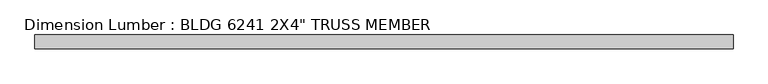
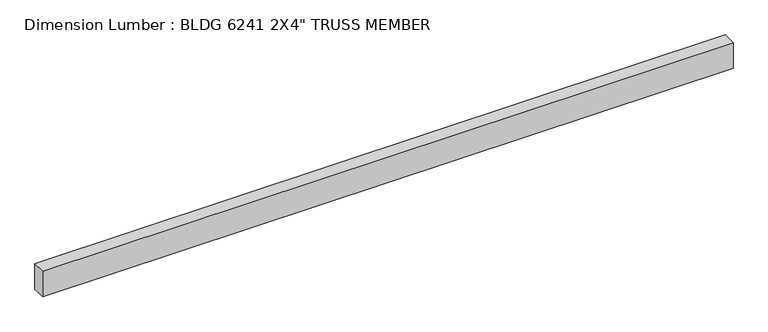
"""IFC4 building model written with IfcOpenShell, lengths in millimetres: beam geometry."""

from ifc_helpers import new_model, si_unit, frame, origin, place, context, project, spatial, polyline, outline, extrude, source, transform, mapped, element, save


def beam_d1363b41(model_context):
    return source(origin(), model_context, "Body", "SweptSolid", [
        extrude(outline(polyline([(1292.2249994, 25.4), (1292.2249994, -25.4), (-1292.2249994, -25.4), (-1292.2249994, 25.4), (1292.2249994, 25.4)])), frame((0.0, 0.0, -50.8), z_axis=(0.0, 0.0, 1.0), x_axis=(1.0, 0.0, 0.0)), (0.0, 0.0, 1.0), 101.6),
    ])


if __name__ == "__main__":
    model = new_model("IFC4")
    model_context = context("Model", 3, world=origin())
    ifc_project = project(units=[si_unit("LENGTHUNIT", "METRE", prefix="MILLI")], contexts=[model_context])
    site = spatial("IfcSite", under=ifc_project)
    building = spatial("IfcBuilding", under=site)
    placement = place(None, origin())
    beam_shape = beam_d1363b41(model_context)
    element("IfcBeam", 1, ObjectType="Dimension Lumber : BLDG 6241 2X4\" TRUSS MEMBER", at=placement, inside=building, context=model_context, shape_type="MappedRepresentation", body=[
        mapped(beam_shape, transform((0.0, 0.0, 0.0), x_axis=(1.0, 0.0, 0.0), y_axis=(0.0, 1.0, 0.0), z_axis=(0.0, 0.0, 1.0))),
    ])
    save(model, "model.ifc")

# Revit data of these elements
# Type "Dimension Lumber : BLDG 6241 2X4\" TRUSS MEMBER"
#   Assembly Code = "B10"
#   A = 0.273472 SF
#   Length [instance default] = 5' - 0"
#   b = 0' - 2"
#   d = 0' - 4"
#   Structural Material [instance default] = Softwood, Lumber
# Element 1 (IfcBeam, "Dimension Lumber : BLDG 6241 2X4\" TRUSS MEMBER")
#   Materials on its faces: "Softwood, Lumber"
# Materials
#   "Softwood, Lumber": class "Wood", colour RGB 223 192 134, transparency 0, Description = "Pinus Echinata", Cost = 0
